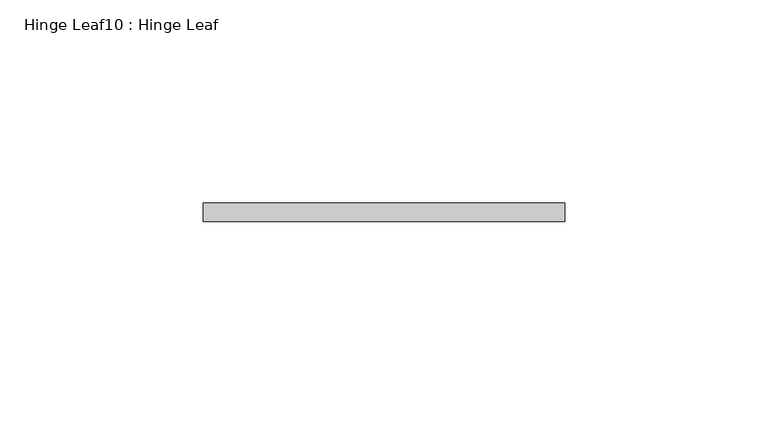
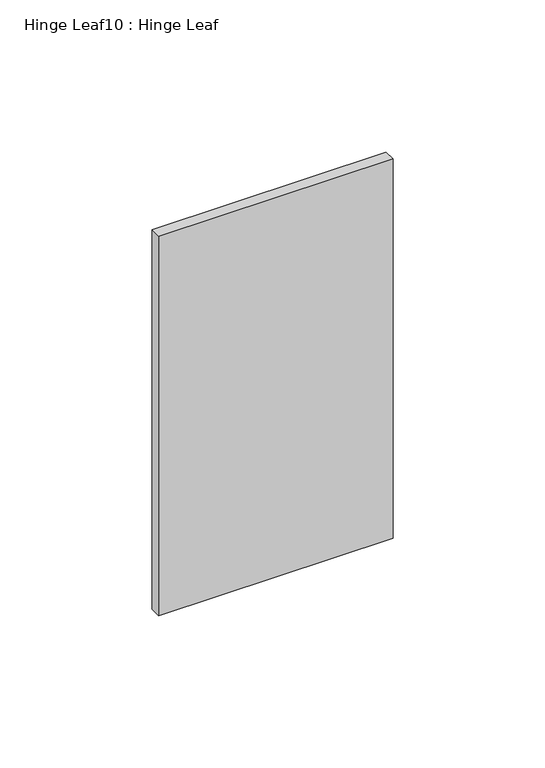
"""IFC4 building model written with IfcOpenShell, lengths in millimetres: proxy geometry, Hinge Leaf10 : Hinge Leaf."""

from ifc_helpers import new_model, si_unit, frame, origin, place, context, project, spatial, polyline, outline, extrude, source, transform, mapped, element, save


def hinge_leaf10_hinge_leaf_a1326aa5(model_context):
    return source(origin(), model_context, "Body", "SweptSolid", [
        extrude(outline(polyline([(587327.7934739, -531780.6943841), (587416.6934739, -531780.6943841), (587416.6934739, -531785.2663841), (587327.7934739, -531785.2663841), (587327.7934739, -531780.6943841)])), frame((0.0, 0.0, 1123.95), z_axis=(0.0, 0.0, 1.0), x_axis=(1.0, 0.0, 0.0)), (0.0, 0.0, 1.0), 152.4),
    ])


if __name__ == "__main__":
    model = new_model("IFC4")
    model_context = context("Model", 3, world=origin())
    ifc_project = project(units=[si_unit("LENGTHUNIT", "METRE", prefix="MILLI")], contexts=[model_context])
    site = spatial("IfcSite", under=ifc_project)
    building = spatial("IfcBuilding", under=site)
    placement = place(None, origin())
    hinge_leaf10_hinge_leaf_shape = hinge_leaf10_hinge_leaf_a1326aa5(model_context)
    element("IfcBuildingElementProxy", 1, Name="Hinge Leaf10 : Hinge Leaf", ObjectType="Hinge Leaf10 : Hinge Leaf", at=placement, inside=building, context=model_context, shape_type="MappedRepresentation", body=[
        mapped(hinge_leaf10_hinge_leaf_shape, transform((0.0, 0.0, 0.0), x_axis=(1.0, 0.0, 0.0), y_axis=(0.0, 1.0, 0.0), z_axis=(0.0, 0.0, 1.0))),
    ])
    save(model, "model.ifc")

# Revit data of these elements
# Element 1 (IfcBuildingElementProxy, "Hinge Leaf10 : Hinge Leaf")
#   Materials on its faces: "6\"X6\" WELD-ON STL BUTT HINGE"
# Materials
#   "6\"X6\" WELD-ON STL BUTT HINGE": class "Metal", colour RGB 189 187 185, transparency 0, Description = "Carbon steel", Cost = 0
